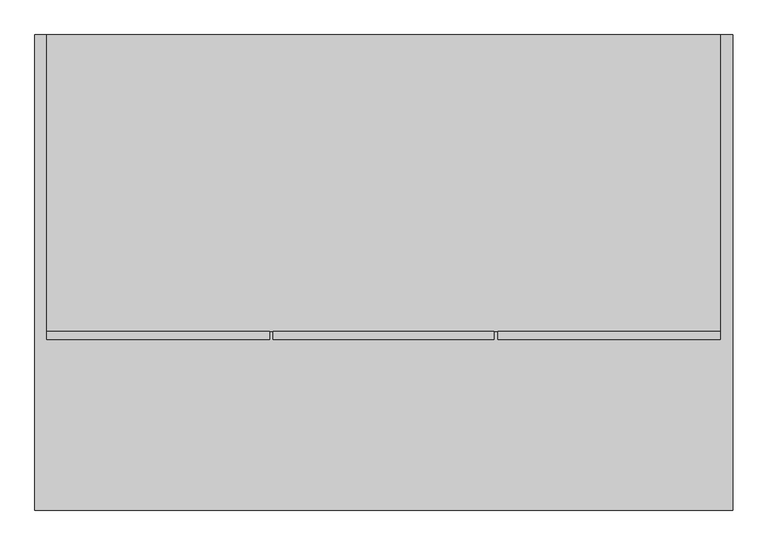
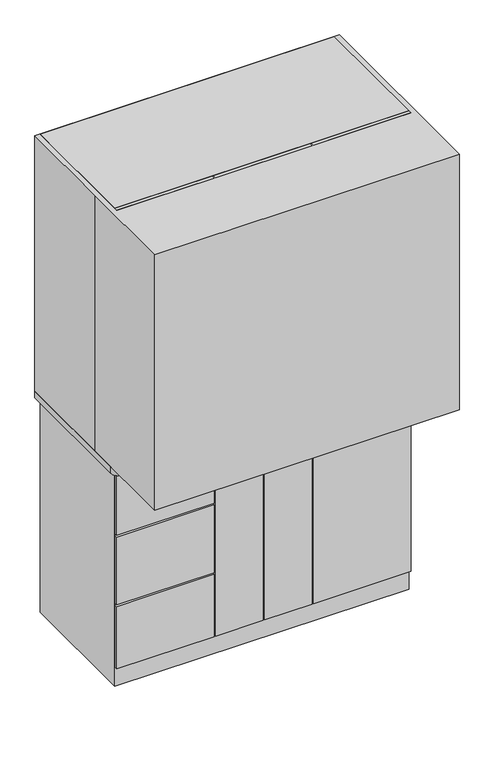
"""IFC4 building model written with IfcOpenShell, lengths in millimetres: proxy geometry, D0670 - Console, Treatment Unit, Dental Operatory : D0670 - Console, Treatment Unit, Dental Operatory."""

import ifcopenshell
import ifcopenshell.guid

model = None  # the IFC model being written
_history = None  # IfcOwnerHistory: only IFC2X3 demands one
_inside = {}  # id of a spatial element -> (the spatial element, [elements in it])
_under = {}  # id of a project, library or spatial element -> (it, [spatial elements below it])
_declared = {}  # id of a project -> (the project, [libraries it declares])
_typed = {}  # id of a type object -> (the type object, [elements of that type])
_made_of = {}  # id of a material, layer set ... -> (it, [elements and type objects made of it])


def new_model(schema):
    """Start an empty IFC model of exactly this schema.

    Asked for "IFC4X3", IfcOpenShell would pick the latest addendum, in which some entities
    have other attributes; the version numbers below select the first issue.
    IFC2X3 requires an IfcOwnerHistory on every rooted entity: one is made here for all.
    """
    global model, _history
    if schema == "IFC4X3":
        model = ifcopenshell.file(schema_version=(4, 3, 0, 0))
    else:
        model = ifcopenshell.file(schema=schema)
    _inside.clear()
    _under.clear()
    _declared.clear()
    _typed.clear()
    _made_of.clear()
    _history = None
    if model.schema == "IFC2X3":
        org = make("IfcOrganization", Name="unknown")
        user = make(
            "IfcPersonAndOrganization",
            ThePerson=make("IfcPerson", FamilyName="unknown"),
            TheOrganization=org,
        )
        app = make(
            "IfcApplication",
            ApplicationDeveloper=org,
            Version="unknown",
            ApplicationFullName="unknown",
            ApplicationIdentifier="unknown",
        )
        _history = make(
            "IfcOwnerHistory",
            OwningUser=user,
            OwningApplication=app,
            ChangeAction="ADDED",
            CreationDate=0,
        )
    return model


def make(cls, **values):
    """One entity of the class cls with the attributes given. An attribute that is None is left unset."""
    return model.create_entity(
        cls, **{name: value for name, value in values.items() if value is not None}
    )


def rooted(cls, **values):
    """An entity with a GlobalId (a new one), such as an element, a storey or a relation."""
    return make(cls, GlobalId=ifcopenshell.guid.new(), OwnerHistory=_history, **values)


def si_unit(unit_type, name, prefix=None):
    """IfcSIUnit, for example si_unit("LENGTHUNIT", "METRE", prefix="MILLI")."""
    return make("IfcSIUnit", UnitType=unit_type, Prefix=prefix, Name=name)


def assignment(units):
    """IfcUnitAssignment: the units of a project."""
    return None if units is None else make("IfcUnitAssignment", Units=units)


def point(xyz):
    """IfcCartesianPoint."""
    return None if xyz is None else make("IfcCartesianPoint", Coordinates=xyz)


def direction(xyz):
    """IfcDirection."""
    return None if xyz is None else make("IfcDirection", DirectionRatios=xyz)


def frame(location, z_axis=None, x_axis=None):
    """IfcAxis2Placement3D, a coordinate frame: its origin and axes. An axis left out is left unset."""
    return make(
        "IfcAxis2Placement3D",
        Location=point(location),
        Axis=direction(z_axis),
        RefDirection=direction(x_axis),
    )


def frame_2d(location, x_axis=None):
    """IfcAxis2Placement2D, a coordinate frame in the plane: its origin and x axis."""
    return make(
        "IfcAxis2Placement2D", Location=point(location), RefDirection=direction(x_axis)
    )


def origin():
    """The frame at (0, 0, 0) with its axes left unset."""
    return frame((0.0, 0.0, 0.0))


def origin_with_axes():
    """The frame at (0, 0, 0) with the z axis (0, 0, 1) and the x axis (1, 0, 0) written out."""
    return frame((0.0, 0.0, 0.0), z_axis=(0.0, 0.0, 1.0), x_axis=(1.0, 0.0, 0.0))


def place(relative_to, where):
    """IfcLocalPlacement: puts the frame where relative to a parent placement (None: the world)."""
    return make(
        "IfcLocalPlacement", PlacementRelTo=relative_to, RelativePlacement=where
    )


def context(
    kind, dimensions, precision=None, world=None, true_north=None, identifier=None
):
    """IfcGeometricRepresentationContext, for example the 3D "Model" context."""
    return make(
        "IfcGeometricRepresentationContext",
        ContextIdentifier=identifier,
        ContextType=kind,
        CoordinateSpaceDimension=dimensions,
        Precision=precision,
        WorldCoordinateSystem=world,
        TrueNorth=true_north,
    )


def project(units=None, contexts=None):
    """IfcProject with its units and contexts."""
    return rooted(
        "IfcProject",
        Name="project",
        RepresentationContexts=contexts,
        UnitsInContext=assignment(units),
    )


def spatial(cls, under=None, at=None, **own):
    """A site, building, storey or space (cls), placed at a placement, below another one or the project."""
    s = rooted(cls, ObjectPlacement=at, **own)
    if under is not None:
        _under.setdefault(under.id(), (under, []))[1].append(s)
    return s


def polyline(points):
    """IfcPolyline through the points."""
    return make("IfcPolyline", Points=[point(p) for p in points])


def circle_curve(where, radius):
    """IfcCircle in the frame where."""
    return make("IfcCircle", Position=where, Radius=radius)


def trimmed(basis, trim1, trim2, sense, master):
    """IfcTrimmedCurve: the piece of a basis curve between two trims."""
    return make(
        "IfcTrimmedCurve",
        BasisCurve=basis,
        Trim1=trim1,
        Trim2=trim2,
        SenseAgreement=sense,
        MasterRepresentation=master,
    )


def segment(curve, same_sense, transition):
    """IfcCompositeCurveSegment."""
    return make(
        "IfcCompositeCurveSegment",
        Transition=transition,
        SameSense=same_sense,
        ParentCurve=curve,
    )


def composite_curve(segments, self_intersect=None):
    """IfcCompositeCurve: segments joined end to end."""
    return make("IfcCompositeCurve", Segments=segments, SelfIntersect=self_intersect)


def outline(outer, holes=None, kind="AREA"):
    """IfcArbitraryClosedProfileDef: a profile drawn as a closed curve; with holes, ...WithVoids."""
    if holes is None:
        return make("IfcArbitraryClosedProfileDef", ProfileType=kind, OuterCurve=outer)
    return make(
        "IfcArbitraryProfileDefWithVoids",
        ProfileType=kind,
        OuterCurve=outer,
        InnerCurves=holes,
    )


def extrude(swept, where, along, depth):
    """IfcExtrudedAreaSolid: the profile swept, set in the frame where, extruded along a direction by depth."""
    return make(
        "IfcExtrudedAreaSolid",
        SweptArea=swept,
        Position=where,
        ExtrudedDirection=direction(along),
        Depth=depth,
    )


def shape(context_of_items, identifier, shape_type, items):
    """IfcShapeRepresentation: the items that make up one representation, for example the "Body"."""
    return make(
        "IfcShapeRepresentation",
        ContextOfItems=context_of_items,
        RepresentationIdentifier=identifier,
        RepresentationType=shape_type,
        Items=items,
    )


def source(mapping_origin, context_of_items, identifier, shape_type, items):
    """IfcRepresentationMap: a shape defined once, which mapped items show again and again."""
    return make(
        "IfcRepresentationMap",
        MappingOrigin=mapping_origin,
        MappedRepresentation=shape(context_of_items, identifier, shape_type, items),
    )


def transform(
    local_origin,
    x_axis=None,
    y_axis=None,
    z_axis=None,
    scale=None,
    scale2=None,
    scale3=None,
    uniform=True,
):
    """IfcCartesianTransformationOperator3D, or its non-uniform kind. x_axis, y_axis, z_axis: its Axis1, 2, 3."""
    if uniform:
        return make(
            "IfcCartesianTransformationOperator3D",
            Axis1=direction(x_axis),
            Axis2=direction(y_axis),
            LocalOrigin=point(local_origin),
            Scale=scale,
            Axis3=direction(z_axis),
        )
    return make(
        "IfcCartesianTransformationOperator3DnonUniform",
        Axis1=direction(x_axis),
        Axis2=direction(y_axis),
        LocalOrigin=point(local_origin),
        Scale=scale,
        Axis3=direction(z_axis),
        Scale2=scale2,
        Scale3=scale3,
    )


def mapped(mapping_source, mapping_target):
    """IfcMappedItem: shows the shape of a source again, moved by a transform."""
    return make(
        "IfcMappedItem", MappingSource=mapping_source, MappingTarget=mapping_target
    )


def made_of(thing, what):
    """Note that an element or type object is made of a material, layer set ...; save() writes the relation."""
    if what is not None:
        _made_of.setdefault(what.id(), (what, []))[1].append(thing)
    return thing


def element(
    cls,
    number,
    at=None,
    inside=None,
    cuts=None,
    type_object=None,
    material=None,
    context=None,
    identifier="Body",
    shape_type=None,
    held_by="IfcProductDefinitionShape",
    body=None,
    shapes=None,
    **own,
):
    """One element of the class cls, such as IfcWall. Its Tag is "e" and its number.

    at: its placement. inside: the storey or other place that contains it. cuts: it is an
    opening in that element (IfcRelVoidsElement). A single representation is given by context,
    identifier, shape_type and body (its items); several are given by shapes. held_by: the class
    of the entity that holds the representations. save() writes the other relations.
    """
    e = rooted(cls, Tag="e%d" % number, ObjectPlacement=at, **own)
    if body is not None:
        shapes = [shape(context, identifier, shape_type, body)]
    if shapes is not None:
        e.Representation = make(held_by, Representations=shapes)
    if inside is not None:
        _inside.setdefault(inside.id(), (inside, []))[1].append(e)
    if cuts is not None:
        rooted(
            "IfcRelVoidsElement", RelatingBuildingElement=cuts, RelatedOpeningElement=e
        )
    if type_object is not None:
        _typed.setdefault(type_object.id(), (type_object, []))[1].append(e)
    return made_of(e, material)


def aggregate(whole, parts):
    """IfcRelAggregates: a whole, such as a stair, and the parts it consists of."""
    return rooted("IfcRelAggregates", RelatingObject=whole, RelatedObjects=parts)


def save(model, path):
    """Write the relations noted so far, then the file.

    IfcRelAggregates (storeys below a building ...), IfcRelContainedInSpatialStructure (elements
    in a storey), IfcRelDefinesByType, IfcRelAssociatesMaterial and IfcRelDeclares: one each for
    every whole, place, type object, material and project.
    """
    for whole, parts in _under.values():
        aggregate(whole, parts)
    for where, things in _inside.values():
        rooted(
            "IfcRelContainedInSpatialStructure",
            RelatedElements=things,
            RelatingStructure=where,
        )
    for kind, things in _typed.values():
        rooted("IfcRelDefinesByType", RelatedObjects=things, RelatingType=kind)
    for what, things in _made_of.values():
        rooted("IfcRelAssociatesMaterial", RelatedObjects=things, RelatingMaterial=what)
    for by, libraries in _declared.values():
        rooted("IfcRelDeclares", RelatingContext=by, RelatedDefinitions=libraries)
    model.write(path)


def specialty_equipment_3eb56f56(model_context):
    return source(origin(), model_context, "Body", "SweptSolid", [
        extrude(outline(composite_curve([segment(polyline([(1692.275, -412.3025692), (1482.725, -412.3025692)]), True, "CONTINUOUS"), segment(trimmed(circle_curve(frame_2d((1482.725, -361.5025692)), 50.8), [point((1482.725, -412.3025692))], [point((1482.725, -310.7025692))], False, "CARTESIAN"), True, "CONTINUOUS"), segment(polyline([(1482.725, -310.7025692), (1692.275, -310.7025692)]), True, "CONTINUOUS"), segment(trimmed(circle_curve(frame_2d((1692.275, -361.5025692)), 50.8), [point((1692.275, -310.7025692))], [point((1692.275, -412.3025692))], False, "CARTESIAN"), True, "CONTINUOUS")], self_intersect=False)), frame((0.0, -106.6936289, 0.0), z_axis=(0.0, 1.0, 0.0), x_axis=(0.0, 0.0, 1.0)), (0.0, 0.0, 1.0), 12.7),
        extrude(outline(composite_curve([segment(trimmed(circle_curve(frame_2d((1482.725, -0.2452076)), 50.8), [point((1482.725, -51.0452076))], [point((1482.725, 50.5547924))], False, "CARTESIAN"), True, "CONTINUOUS"), segment(polyline([(1482.725, 50.5547924), (1692.275, 50.5547924)]), True, "CONTINUOUS"), segment(trimmed(circle_curve(frame_2d((1692.275, -0.2452076)), 50.8), [point((1692.275, 50.5547924))], [point((1692.275, -51.0452076))], False, "CARTESIAN"), True, "CONTINUOUS"), segment(polyline([(1692.275, -51.0452076), (1482.725, -51.0452076)]), True, "CONTINUOUS")], self_intersect=False)), frame((0.0, -106.6936289, 0.0), z_axis=(0.0, 1.0, 0.0), x_axis=(0.0, 0.0, 1.0)), (0.0, 0.0, 1.0), 12.7),
        extrude(outline(composite_curve([segment(polyline([(1692.275, 310.212154), (1482.725, 310.212154)]), True, "CONTINUOUS"), segment(trimmed(circle_curve(frame_2d((1482.725, 361.012154)), 50.8), [point((1482.725, 310.212154))], [point((1482.725, 411.812154))], False, "CARTESIAN"), True, "CONTINUOUS"), segment(polyline([(1482.725, 411.812154), (1692.275, 411.812154)]), True, "CONTINUOUS"), segment(trimmed(circle_curve(frame_2d((1692.275, 361.012154)), 50.8), [point((1692.275, 411.812154))], [point((1692.275, 310.212154))], False, "CARTESIAN"), True, "CONTINUOUS")], self_intersect=False)), frame((0.0, -106.6936289, 0.0), z_axis=(0.0, 1.0, 0.0), x_axis=(0.0, 0.0, 1.0)), (0.0, 0.0, 1.0), 12.7),
        extrude(outline(polyline([(1854.2, -183.2551384), (1854.2, -539.75), (1320.8, -539.75), (1320.8, -183.2551384), (1854.2, -183.2551384)]), holes=[composite_curve([segment(trimmed(circle_curve(frame_2d((1692.275, -361.5025692)), 50.8), [point((1692.275, -412.3025692))], [point((1692.275, -310.7025692))], True, "CARTESIAN"), True, "CONTINUOUS"), segment(polyline([(1692.275, -310.7025692), (1482.725, -310.7025692)]), True, "CONTINUOUS"), segment(trimmed(circle_curve(frame_2d((1482.725, -361.5025692)), 50.8), [point((1482.725, -310.7025692))], [point((1482.725, -412.3025692))], True, "CARTESIAN"), True, "CONTINUOUS"), segment(polyline([(1482.725, -412.3025692), (1692.275, -412.3025692)]), True, "CONTINUOUS")], self_intersect=False)]), frame((0.0, -106.6936289, 0.0), z_axis=(0.0, 1.0, 0.0), x_axis=(0.0, 0.0, 1.0)), (0.0, 0.0, 1.0), 12.7),
        extrude(outline(polyline([(1854.2, -176.9051384), (1320.8, -176.9051384), (1320.8, 176.4147232), (1854.2, 176.4147232), (1854.2, -176.9051384)]), holes=[composite_curve([segment(trimmed(circle_curve(frame_2d((1692.275, -0.2452076)), 50.8), [point((1692.275, -51.0452076))], [point((1692.275, 50.5547924))], True, "CARTESIAN"), True, "CONTINUOUS"), segment(polyline([(1692.275, 50.5547924), (1482.725, 50.5547924)]), True, "CONTINUOUS"), segment(trimmed(circle_curve(frame_2d((1482.725, -0.2452076)), 50.8), [point((1482.725, 50.5547924))], [point((1482.725, -51.0452076))], True, "CARTESIAN"), True, "CONTINUOUS"), segment(polyline([(1482.725, -51.0452076), (1692.275, -51.0452076)]), True, "CONTINUOUS")], self_intersect=False)]), frame((0.0, -106.6936289, 0.0), z_axis=(0.0, 1.0, 0.0), x_axis=(0.0, 0.0, 1.0)), (0.0, 0.0, 1.0), 12.7),
        extrude(outline(polyline([(1854.2, 182.7647232), (1320.8, 182.7647232), (1320.8, 539.2595848), (1854.2, 539.2595848), (1854.2, 182.7647232)]), holes=[composite_curve([segment(trimmed(circle_curve(frame_2d((1692.275, 361.012154)), 50.8), [point((1692.275, 310.212154))], [point((1692.275, 411.812154))], True, "CARTESIAN"), True, "CONTINUOUS"), segment(polyline([(1692.275, 411.812154), (1482.725, 411.812154)]), True, "CONTINUOUS"), segment(trimmed(circle_curve(frame_2d((1482.725, 361.012154)), 50.8), [point((1482.725, 411.812154))], [point((1482.725, 310.212154))], True, "CARTESIAN"), True, "CONTINUOUS"), segment(polyline([(1482.725, 310.212154), (1692.275, 310.212154)]), True, "CONTINUOUS")], self_intersect=False)]), frame((0.0, -106.6936289, 0.0), z_axis=(0.0, 1.0, 0.0), x_axis=(0.0, 0.0, 1.0)), (0.0, 0.0, 1.0), 12.7),
        extrude(outline(polyline([(-183.2551384, -106.6936289), (-539.75, -106.6936289), (-539.75, -93.9936289), (-183.2551384, -93.9936289), (-183.2551384, -106.6936289)])), frame((0.0, 0.0, 593.725), z_axis=(0.0, 0.0, 1.0), x_axis=(1.0, 0.0, 0.0)), (0.0, 0.0, 1.0), 244.475),
        extrude(outline(polyline([(-183.2551384, -106.6936289), (-539.75, -106.6936289), (-539.75, -93.9936289), (-183.2551384, -93.9936289), (-183.2551384, -106.6936289)])), frame((0.0, 0.0, 76.2600653), z_axis=(0.0, 0.0, 1.0), x_axis=(1.0, 0.0, 0.0)), (0.0, 0.0, 1.0), 241.2399347),
        extrude(outline(polyline([(539.2595848, -106.6936289), (182.7647232, -106.6936289), (182.7647232, -93.9936289), (539.2595848, -93.9936289), (539.2595848, -106.6936289)])), frame((0.0, 0.0, 76.2600653), z_axis=(0.0, 0.0, 1.0), x_axis=(1.0, 0.0, 0.0)), (0.0, 0.0, 1.0), 761.9399347),
        extrude(outline(polyline([(-3.4202076, -106.6936289), (-176.9051384, -106.6936289), (-176.9051384, -93.9936289), (-3.4202076, -93.9936289), (-3.4202076, -106.6936289)])), frame((0.0, 0.0, 76.2600653), z_axis=(0.0, 0.0, 1.0), x_axis=(1.0, 0.0, 0.0)), (0.0, 0.0, 1.0), 761.9399347),
        extrude(outline(polyline([(176.4147232, -106.6936289), (2.9297924, -106.6936289), (2.9297924, -93.9936289), (176.4147232, -93.9936289), (176.4147232, -106.6936289)])), frame((0.0, 0.0, 76.2600653), z_axis=(0.0, 0.0, 1.0), x_axis=(1.0, 0.0, 0.0)), (0.0, 0.0, 1.0), 761.9399347),
        extrude(outline(polyline([(-183.2551384, -106.6936289), (-539.75, -106.6936289), (-539.75, -93.9936289), (-183.2551384, -93.9936289), (-183.2551384, -106.6936289)])), frame((0.0, 0.0, 323.85), z_axis=(0.0, 0.0, 1.0), x_axis=(1.0, 0.0, 0.0)), (0.0, 0.0, 1.0), 263.525),
        extrude(outline(polyline([(513.8595848, 355.6), (-514.35, 355.6), (-514.35, 381.0), (513.8595848, 381.0), (513.8595848, 355.6)])), frame((0.0, 0.0, 863.6), z_axis=(0.0, 0.0, 1.0), x_axis=(1.0, 0.0, 0.0)), (0.0, 0.0, 1.0), 381.0),
        extrude(outline(polyline([(-514.35, 203.2), (-539.75, 203.2), (-539.75, 381.0), (-514.35, 381.0), (-514.35, 203.2)])), frame((0.0, 0.0, 863.6), z_axis=(0.0, 0.0, 1.0), x_axis=(1.0, 0.0, 0.0)), (0.0, 0.0, 1.0), 381.0),
        extrude(outline(polyline([(539.2595848, 203.2), (513.8595848, 203.2), (513.8595848, 381.0), (539.2595848, 381.0), (539.2595848, 203.2)])), frame((0.0, 0.0, 863.6), z_axis=(0.0, 0.0, 1.0), x_axis=(1.0, 0.0, 0.0)), (0.0, 0.0, 1.0), 381.0),
        extrude(outline(composite_curve([segment(polyline([(-558.8, -101.6), (-558.8, 381.0), (558.8, 381.0), (558.8, -101.6)]), True, "CONTINUOUS"), segment(trimmed(circle_curve(frame_2d((533.4, -101.6)), 25.4), [point((558.8, -101.6))], [point((533.4, -127.0))], False, "CARTESIAN"), True, "CONTINUOUS"), segment(polyline([(533.4, -127.0), (-533.4, -127.0)]), True, "CONTINUOUS"), segment(trimmed(circle_curve(frame_2d((-533.4, -101.6)), 25.4), [point((-533.4, -127.0))], [point((-558.8, -101.6))], False, "CARTESIAN"), True, "CONTINUOUS")], self_intersect=False)), frame((0.0, 0.0, 838.2), z_axis=(0.0, 0.0, 1.0), x_axis=(1.0, 0.0, 0.0)), (0.0, 0.0, 1.0), 25.4),
        extrude(outline(polyline([(539.2595848, 381.0), (539.2595848, -93.9936289), (-539.75, -93.9936289), (-539.75, 381.0), (539.2595848, 381.0)])), frame((0.0, 0.0, 1244.6), z_axis=(0.0, 0.0, 1.0), x_axis=(1.0, 0.0, 0.0)), (0.0, 0.0, 1.0), 609.6),
        extrude(outline(polyline([(539.2595848, 381.0), (539.2595848, -93.9936289), (-539.75, -93.9936289), (-539.75, 381.0), (539.2595848, 381.0)])), origin_with_axes(), (0.0, 0.0, 1.0), 838.2),
        extrude(outline(polyline([(-558.8, 381.0), (558.8, 381.0), (558.8, -381.0), (-558.8, -381.0), (-558.8, 0.0), (-558.8, 381.0)])), frame((0.0, 0.0, 863.6), z_axis=(0.0, 0.0, 1.0), x_axis=(1.0, 0.0, 0.0)), (0.0, 0.0, 1.0), 990.6),
    ])


if __name__ == "__main__":
    model = new_model("IFC4")
    model_context = context("Model", 3, world=origin())
    ifc_project = project(units=[si_unit("LENGTHUNIT", "METRE", prefix="MILLI")], contexts=[model_context])
    site = spatial("IfcSite", under=ifc_project)
    building = spatial("IfcBuilding", under=site)
    placement = place(None, origin())
    specialty_equipment_shape = specialty_equipment_3eb56f56(model_context)
    element("IfcBuildingElementProxy", 1, Name="D0670 - Console, Treatment Unit, Dental Operatory : D0670 - Console, Treatment Unit, Dental Operatory", ObjectType="D0670 - Console, Treatment Unit, Dental Operatory : D0670 - Console, Treatment Unit, Dental Operatory", at=placement, inside=building, context=model_context, shape_type="MappedRepresentation", body=[
        mapped(specialty_equipment_shape, transform((0.0, 0.0, 0.0), x_axis=(1.0, 0.0, 0.0), y_axis=(0.0, 1.0, 0.0), z_axis=(0.0, 0.0, 1.0))),
    ])
    save(model, "model.ifc")

# Revit data of these elements
# Project information
#   Room Abbreviation = "DNTG4"
#   Room Description = "Dental Treatment Room, Multi-Chair (DNTG4)"
#   Sheets - Total = "5"
#   Project Issue Date = "Issue Date"
#   Project Status = "Project Status"
#   Client Name = "Owner"
#   Project Address = "Enter address here"
#   Project Name = "Project Name"
#   Project Number = "Project Number"
#   Publication Date = "1-Feb-16"
# Type "D0670 - Console, Treatment Unit, Dental Operatory : D0670 - Console, Treatment Unit, Dental Operatory"
#   Watts2 = "0"
#   Watts1 = "240"
#   Unit_Issue = "EA"
#   UTIL_6_Misc = "-"
#   UTIL_5_NonMedGas = "-"
#   UTIL_4_MiscGas = "-"
#   UTIL_3_MedGas = "-"
#   UTIL_2_Elec = "A"
#   UTIL_1_WaterDrain = "D"
#   Nomenclature = "Console, Treatment Unit, Dental Operatory"
#   NSN = "6520"
#   Location [instance default] = ""
#   JSN = "D0670"
#   Fund_Source_VA = "-"
#   Fund_Source_Navy = "-"
#   Fund_Source_Army = "-"
#   Fund_Source_AF = "-"
#   ELEC_Volts2 = "0"
#   ELEC_Volts1 = "120"
#   ELEC_Phase2 = "0"
#   ELEC_Phase1 = "1"
#   ELEC_HertzSwitch = "0"
#   ELEC_HertzDependent = "0"
#   ELEC_Hertz = "60"
#   ELEC_Amps2 = "0"
#   ELEC_Amps1 = "2"
#   DetailDescription = "A dental treatment console or work station (also called a \"12 o'clock unit) approximately 45\" W x 72\" H x 30\" D. Consists of a base unit with storage and equipment drawers, a bifold door cabinet with slide out shelves and CPU storage. A  midsection with chase and power bar for ancillary equipment and shelf for a monitor and keyboard. Upper storage unit may be pass-through or non-pass-through with glass shelves and see-through cabinet doors. Unit may also be configured with a pivoting work surface to hold all doctor and assistant instrumentation or with a wash station w/SS sink and knee or foot activated faucet and solid surface or laminate countertop. Unit is also available in other widths and heights. Final makeup of this unit is dependant on individual facility requirements determined at time of purchase."
#   CAT_VA = "A"
#   CAT_Navy = "A"
#   CAT_IHS = "-"
#   CAT_Army = "A"
#   CAT_AF = "A"
#   BTUperhour = "0"
#   Weight_IP = 0
#   DIM_Width_IP = 3' - 8"
#   DIM_Height_IP = 6' - 1"
#   DIM_Depth_IP = 2' - 6"
# Element 1 (IfcBuildingElementProxy, "D0670 - Console, Treatment Unit, Dental Operatory : D0670 - Console, Treatment Unit, Dental Operatory")
#   Materials on its faces: "Glass", "EquipSpace"
# Materials
#   "Glass": class "Glass", colour RGB 0 128 192, transparency 0.75
#   "EquipSpace": class "Unassigned", colour RGB 221 217 195, transparency 0.5
